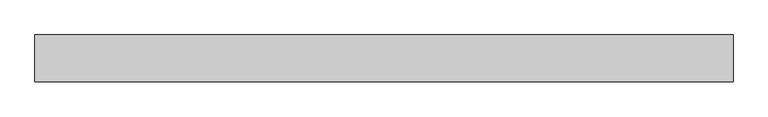
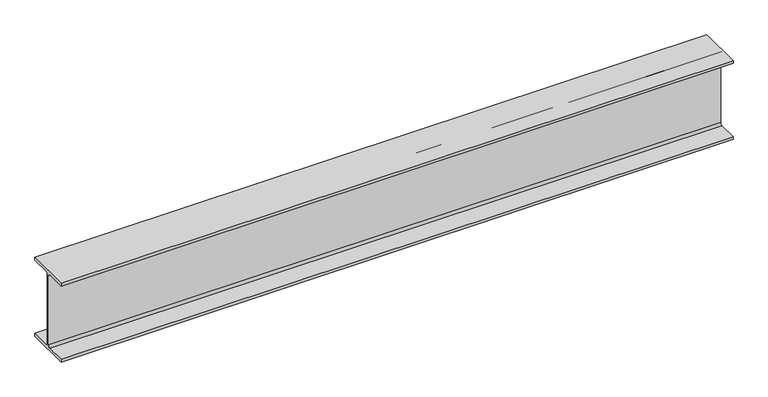
"""IFC4 building model written with IfcOpenShell, lengths in millimetres: beam geometry, Old_Steel Beam_H-KSD3502 : H_SB_ASB_H-194×150x6x9."""

from ifc_helpers import new_model, si_unit, point, frame, frame_2d, origin, place, context, project, spatial, polyline, circle_curve, trimmed, segment, composite_curve, outline, extrude, source, transform, mapped, element, save


def beam_59e108a4(model_context):
    return source(origin(), model_context, "Body", "SweptSolid", [
        extrude(outline(composite_curve([segment(polyline([(82.5, -141.5), (82.5, -151.7), (-82.5, -151.7), (-82.5, -141.5), (-11.9, -141.5)]), True, "CONTINUOUS"), segment(trimmed(circle_curve(frame_2d((-11.9, -132.6)), 8.9), [point((-11.9, -141.5))], [point((-3.0, -132.6))], True, "CARTESIAN"), True, "CONTINUOUS"), segment(polyline([(-3.0, -132.6), (-3.0, 132.6)]), True, "CONTINUOUS"), segment(trimmed(circle_curve(frame_2d((-11.9, 132.6)), 8.9), [point((-3.0, 132.6))], [point((-11.9, 141.5))], True, "CARTESIAN"), True, "CONTINUOUS"), segment(polyline([(-11.9, 141.5), (-82.5, 141.5), (-82.5, 151.7), (82.5, 151.7), (82.5, 141.5), (11.9, 141.5)]), True, "CONTINUOUS"), segment(trimmed(circle_curve(frame_2d((11.9, 132.6)), 8.9), [point((11.9, 141.5))], [point((3.0, 132.6))], True, "CARTESIAN"), True, "CONTINUOUS"), segment(polyline([(3.0, 132.6), (3.0, -132.6)]), True, "CONTINUOUS"), segment(trimmed(circle_curve(frame_2d((11.9, -132.6)), 8.9), [point((3.0, -132.6))], [point((11.9, -141.5))], True, "CARTESIAN"), True, "CONTINUOUS"), segment(polyline([(11.9, -141.5), (82.5, -141.5)]), True, "CONTINUOUS")], self_intersect=False)), frame((-1200.0, 0.0, 0.0), z_axis=(1.0, 0.0, 0.0), x_axis=(0.0, 1.0, 0.0)), (0.0, 0.0, 1.0), 2453.1701073),
    ])


if __name__ == "__main__":
    model = new_model("IFC4")
    model_context = context("Model", 3, world=origin())
    ifc_project = project(units=[si_unit("LENGTHUNIT", "METRE", prefix="MILLI")], contexts=[model_context])
    site = spatial("IfcSite", under=ifc_project)
    building = spatial("IfcBuilding", under=site)
    placement = place(None, origin())
    beam_shape = beam_59e108a4(model_context)
    element("IfcBeam", 1, ObjectType="Old_Steel Beam_H-KSD3502 : H_SB_ASB_H-194×150x6x9", at=placement, inside=building, context=model_context, shape_type="MappedRepresentation", body=[
        mapped(beam_shape, transform((0.0, 0.0, 0.0), x_axis=(1.0, 0.0, 0.0), y_axis=(0.0, 1.0, 0.0), z_axis=(0.0, 0.0, 1.0))),
    ])
    save(model, "model.ifc")

# Revit data of these elements
# Type "Old_Steel Beam_H-KSD3502 : H_SB_ASB_H-194×150x6x9"
#   Width = 15.0 cm
#   Web Thickness = 0.6 cm
#   Web Fillet = 1.3 cm
#   Warping Constant = 43316.0 cm⁶
#   Torsional Moment of Inertia = 8.622 cm⁴
#   Torsional Modulus = 1.0 cm³
#   Section Area = 39.01 cm²
#   Plastic Modulus weak axis = 104.0 cm³
#   Plastic Modulus strong axis = 309.0 cm³
#   Perimeter = 0.95 m²/m
#   Nominal Weight = 30.60 kgf/m
#   Moment of Inertia weak axis = 507.00 cm⁴
#   Moment of Inertia strong axis = 2690.00 cm⁴
#   Height = 19.4 cm
#   Flange Thickness = 0.9 cm
#   Elastic Modulus weak axis = 67.6 cm³
#   Elastic Modulus strong axis = 277.0 cm³
#   Centroid Vertical = 9.7 cm
#   Centroid Horizontal = 7.5 cm
#   Length [instance default] = 1.5240 m
#   Structural Material [instance default] = Steel, 45-345
#   Assembly Code = ""
# Element 1 (IfcBeam, "Old_Steel Beam_H-KSD3502 : H_SB_ASB_H-194×150x6x9")
#   Structural Material = none
# Materials
#   "Steel, 45-345": class "Metal", colour RGB 189 187 185, transparency 0, Description = "Steel 345 MPa", Cost = 0
